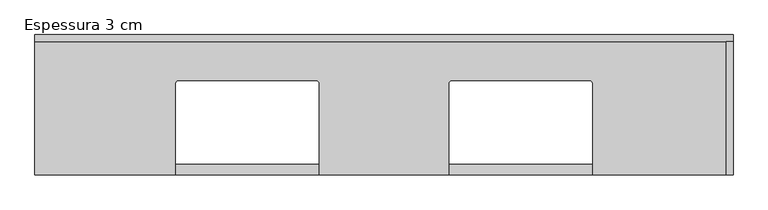
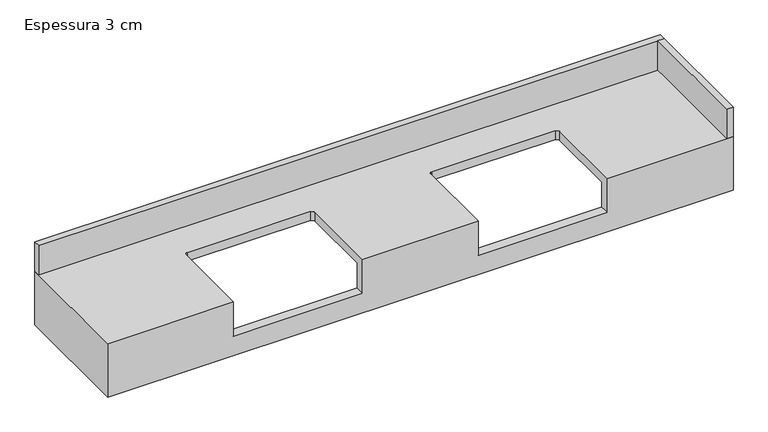
"""IFC4 building model written with IfcOpenShell, lengths in millimetres: furniture geometry, CC_BANCADA BANHEIRO COM DUAS CUBAS_CANTO RETO : Espessura 3 cm."""

from ifc_helpers import new_model, si_unit, frame, origin, place, context, project, spatial, polyline, circle_curve, outline, extrude, source, transform, mapped, element, save
from ifc_brep_helpers import plane_surface, revolved_surface, advanced_brep


def espessura_3_cm_cd586bec(model_context):
    return source(origin(), model_context, "Body", "SolidModel", [
        advanced_brep(
        [(750.0, 300.0, 860.0), (-1237.8, 300.0, 860.0), (-1237.8, -100.0, 860.0), (-837.8, -100.0, 860.0), (-837.8, 160.0, 860.0), (-827.8, 170.0, 860.0), (-437.8, 170.0, 860.0), (-427.8, 160.0, 860.0), (-427.8, -100.0, 860.0), (-60.0, -100.0, 860.0), (-60.0, 160.0, 860.0), (-50.0, 170.0, 860.0), (340.0, 170.0, 860.0), (350.0, 160.0, 860.0), (350.0, -100.0, 860.0), (750.0, -100.0, 860.0), (750.0, 300.0, 680.0), (720.0, 300.0, 680.0), (720.0, 300.0, 830.0), (-1207.8, 300.0, 830.0), (-1207.8, 300.0, 680.0), (-1237.8, 300.0, 680.0), (-1237.8, -100.0, 680.0), (750.0, -100.0, 680.0), (350.0, -100.0, 745.0), (-60.0, -100.0, 745.0), (-427.8, -100.0, 745.0), (-837.8, -100.0, 745.0), (720.0, -70.0, 830.0), (350.0, -70.0, 830.0), (350.0, 160.0, 830.0), (340.0, 170.0, 830.0), (-50.0, 170.0, 830.0), (-60.0, 160.0, 830.0), (-60.0, -70.0, 830.0), (-427.8, -70.0, 830.0), (-427.8, 160.0, 830.0), (-437.8, 170.0, 830.0), (-827.8, 170.0, 830.0), (-837.8, 160.0, 830.0), (-837.8, -70.0, 830.0), (-1207.8, -70.0, 830.0), (-1207.8, -70.0, 680.0), (-837.8, -70.0, 745.0), (-427.8, -70.0, 745.0), (-60.0, -70.0, 745.0), (350.0, -70.0, 745.0), (720.0, -70.0, 680.0)],
        [
            (0, 1),
            (1, 2),
            (2, 3),
            (3, 4),
            (4, 5, circle_curve(frame((-827.8, 160.0, 860.0), z_axis=(0.0, 0.0, -1.0), x_axis=(0.0, 1.0, 0.0)), 10.0)),
            (5, 6),
            (6, 7, circle_curve(frame((-437.8, 160.0, 860.0), z_axis=(0.0, 0.0, -1.0), x_axis=(0.0, 1.0, 0.0)), 10.0)),
            (7, 8),
            (8, 9),
            (9, 10),
            (10, 11, circle_curve(frame((-50.0, 160.0, 860.0), z_axis=(0.0, 0.0, -1.0), x_axis=(0.0, 1.0, 0.0)), 10.0)),
            (11, 12),
            (12, 13, circle_curve(frame((340.0, 160.0, 860.0), z_axis=(0.0, 0.0, -1.0), x_axis=(0.0, 1.0, 0.0)), 10.0)),
            (13, 14),
            (14, 15),
            (15, 0),
            (0, 16),
            (16, 17),
            (17, 18),
            (18, 19),
            (19, 20),
            (20, 21),
            (21, 1),
            (21, 22),
            (22, 2),
            (22, 23),
            (23, 15),
            (14, 24),
            (24, 25),
            (25, 9),
            (8, 26),
            (26, 27),
            (27, 3),
            (23, 16),
            (18, 28),
            (28, 29),
            (29, 30),
            (30, 31, circle_curve(frame((340.0, 160.0, 830.0), z_axis=(0.0, 0.0, 1.0), x_axis=(0.0, 1.0, 0.0)), 10.0)),
            (31, 32),
            (32, 33, circle_curve(frame((-50.0, 160.0, 830.0), z_axis=(0.0, 0.0, 1.0), x_axis=(0.0, 1.0, 0.0)), 10.0)),
            (33, 34),
            (34, 35),
            (35, 36),
            (36, 37, circle_curve(frame((-437.8, 160.0, 830.0), z_axis=(0.0, 0.0, 1.0), x_axis=(0.0, 1.0, 0.0)), 10.0)),
            (37, 38),
            (38, 39, circle_curve(frame((-827.8, 160.0, 830.0), z_axis=(0.0, 0.0, 1.0), x_axis=(0.0, 1.0, 0.0)), 10.0)),
            (39, 40),
            (40, 41),
            (41, 19),
            (41, 42),
            (42, 20),
            (40, 43),
            (43, 44),
            (44, 35),
            (34, 45),
            (45, 46),
            (46, 29),
            (28, 47),
            (47, 42),
            (17, 47),
            (5, 38),
            (37, 6),
            (26, 44),
            (43, 27),
            (4, 39),
            (7, 36),
            (24, 46),
            (45, 25),
            (11, 32),
            (31, 12),
            (10, 33),
            (13, 30),
        ],
        [
            plane_surface(frame((-1237.8, 300.0, 860.0), z_axis=(0.0, 0.0, 1.0), x_axis=(-1.0, 0.0, 0.0))),
            plane_surface(frame((750.0, 300.0, 860.0), z_axis=(0.0, 1.0, 0.0), x_axis=(0.0, 0.0, -1.0))),
            plane_surface(frame((-1237.8, 300.0, 860.0), z_axis=(-1.0, 0.0, 0.0), x_axis=(0.0, 0.0, -1.0))),
            plane_surface(frame((-1237.8, -100.0, 860.0), z_axis=(0.0, -1.0, 0.0), x_axis=(0.0, 0.0, -1.0))),
            plane_surface(frame((750.0, -100.0, 860.0), z_axis=(1.0, 0.0, 0.0), x_axis=(0.0, 0.0, -1.0))),
            plane_surface(frame((-1207.8, 300.0, 830.0), z_axis=(0.0, 0.0, -1.0), x_axis=(-1.0, 0.0, 0.0))),
            plane_surface(frame((-1207.8, 300.0, 830.0), z_axis=(1.0, 0.0, 0.0), x_axis=(0.0, 0.0, -1.0))),
            plane_surface(frame((-1207.8, -70.0, 830.0), z_axis=(0.0, 1.0, 0.0), x_axis=(0.0, 0.0, -1.0))),
            plane_surface(frame((720.0, -70.0, 830.0), z_axis=(-1.0, 0.0, 0.0), x_axis=(0.0, 0.0, -1.0))),
            plane_surface(frame((750.0, -100.0, 680.0), z_axis=(0.0, 0.0, -1.0), x_axis=(0.0, 1.0, 0.0))),
            plane_surface(frame((-827.8, 170.0, 745.0), z_axis=(0.0, -1.0, 0.0), x_axis=(0.0, 0.0, 1.0))),
            plane_surface(frame((-437.8, 170.0, 745.0), z_axis=(0.0, 0.0, 1.0), x_axis=(1.0, 0.0, 0.0))),
            revolved_surface(polyline([(-827.8, 170.0, 830.0), (-827.8, 170.0, 860.0)]), (-827.8, 160.0, 900.0), (0.0, 0.0, -1.0)),
            plane_surface(frame((-837.8, -230.0, 745.0), z_axis=(1.0, 0.0, 0.0), x_axis=(0.0, 0.0, 1.0))),
            plane_surface(frame((-427.8, 160.0, 745.0), z_axis=(-1.0, 0.0, 0.0), x_axis=(0.0, 0.0, 1.0))),
            revolved_surface(polyline([(-437.8, 170.0, 830.0), (-437.8, 170.0, 860.0)]), (-437.8, 160.0, 900.0), (0.0, 0.0, -1.0)),
            plane_surface(frame((340.0, 170.0, 745.0), z_axis=(0.0, 0.0, 1.0), x_axis=(1.0, 0.0, 0.0))),
            plane_surface(frame((-50.0, 170.0, 745.0), z_axis=(0.0, -1.0, 0.0), x_axis=(0.0, 0.0, 1.0))),
            revolved_surface(polyline([(-50.0, 170.0, 830.0), (-50.0, 170.0, 860.0)]), (-50.0, 160.0, 900.0), (0.0, 0.0, -1.0)),
            plane_surface(frame((-60.0, -230.0, 745.0), z_axis=(1.0, 0.0, 0.0), x_axis=(0.0, 0.0, 1.0))),
            plane_surface(frame((350.0, 160.0, 745.0), z_axis=(-1.0, 0.0, 0.0), x_axis=(0.0, 0.0, 1.0))),
            revolved_surface(polyline([(340.0, 170.0, 830.0), (340.0, 170.0, 860.0)]), (340.0, 160.0, 900.0), (0.0, 0.0, -1.0)),
        ],
        [
            (0, [[1, 2, 3, 4, 5, 6, 7, 8, 9, 10, 11, 12, 13, 14, 15, 16]]),
            (1, [[-1, 17, 18, 19, 20, 21, 22, 23]]),
            (2, [[-2, -23, 24, 25]]),
            (3, [[-3, -25, 26, 27, -15, 28, 29, 30, -9, 31, 32, 33]]),
            (4, [[-16, -27, 34, -17]]),
            (5, [[35, 36, 37, 38, 39, 40, 41, 42, 43, 44, 45, 46, 47, 48, 49, -20]]),
            (6, [[-49, 50, 51, -21]]),
            (7, [[-48, 52, 53, 54, -42, 55, 56, 57, -36, 58, 59, -50]]),
            (8, [[-35, -19, 60, -58]]),
            (9, [[-18, -34, -26, -24, -22, -51, -59, -60]]),
            (10, [[-6, 61, -45, 62]]),
            (11, [[-32, 63, -53, 64]]),
            (12, [[-5, 65, -46, -61]]),
            (13, [[-4, -33, -64, -52, -47, -65]]),
            (14, [[-8, 66, -43, -54, -63, -31]]),
            (15, [[-7, -62, -44, -66]]),
            (16, [[-29, 67, -56, 68]]),
            (17, [[-12, 69, -39, 70]]),
            (18, [[-11, 71, -40, -69]]),
            (19, [[-10, -30, -68, -55, -41, -71]]),
            (20, [[-14, 72, -37, -57, -67, -28]]),
            (21, [[-13, -70, -38, -72]]),
        ],
    ),
        extrude(outline(polyline([(730.0, 280.0), (750.0, 280.0), (750.0, -100.0), (730.0, -100.0), (730.0, 280.0)])), frame((0.0, 0.0, 860.0), z_axis=(0.0, 0.0, 1.0), x_axis=(1.0, 0.0, 0.0)), (0.0, 0.0, 1.0), 100.0),
        extrude(outline(polyline([(750.0, 300.0), (750.0, 280.0), (-1237.8, 280.0), (-1237.8, 300.0), (750.0, 300.0)])), frame((0.0, 0.0, 860.0), z_axis=(0.0, 0.0, 1.0), x_axis=(1.0, 0.0, 0.0)), (0.0, 0.0, 1.0), 100.0),
    ])


if __name__ == "__main__":
    model = new_model("IFC4")
    model_context = context("Model", 3, world=origin())
    ifc_project = project(units=[si_unit("LENGTHUNIT", "METRE", prefix="MILLI")], contexts=[model_context])
    site = spatial("IfcSite", under=ifc_project)
    building = spatial("IfcBuilding", under=site)
    placement = place(None, origin())
    espessura_3_cm_shape = espessura_3_cm_cd586bec(model_context)
    element("IfcFurniture", 1, ObjectType="CC_BANCADA BANHEIRO COM DUAS CUBAS_CANTO RETO : Espessura 3 cm", at=placement, inside=building, context=model_context, shape_type="MappedRepresentation", body=[
        mapped(espessura_3_cm_shape, transform((0.0, 0.0, 0.0), x_axis=(1.0, 0.0, 0.0), y_axis=(0.0, 1.0, 0.0), z_axis=(0.0, 0.0, 1.0))),
    ])
    save(model, "model.ifc")

# Revit data of these elements
# Type "CC_BANCADA BANHEIRO COM DUAS CUBAS_CANTO RETO : Espessura 3 cm"
#   Uso HS [instance default] = ""
#   h TESTEIRA AUX [instance default] = 0.15 m
#   Altura testeira [instance default] = 0.15 m
#   Altura rodapia [instance default] = 0.10 m
#   Espessura rodapia [instance default] = 0.02 m
#   Prof/2 [instance default] = 0.20 m
#   Offset cuba direita [instance default] = 0.40 m
#   Offset cuba esquerda [instance default] = 0.40 m
#   Depth [instance default] = 2.00 m
#   Width [instance default] = 0.40 m
#   Espessura bancada = 0.03 m
#   Comprimento [instance default] = 2.00 m
#   Height [instance default] = 0.86 m
#   Testeira [instance default] = yes
#   Rodapia fundo [instance default] = no
#   Rodapia esquerda [instance default] = no
#   Rodapia direita [instance default] = no
#   Material porta-toalha [instance default] = .CROMADO
#   Material hidráulico [instance default] = .CROMADO
#   Material cuba [instance default] = .PORCELANA BRANCA
#   Material bancada [instance default] = .GRANITO_BRANCO_ITAUNAS
#   Assembly Code = ""
# Element 1 (IfcFurniture, "CC_BANCADA BANHEIRO COM DUAS CUBAS_CANTO RETO : Espessura 3 cm")
#   Uso HS = "SUÍTE MASTER"
#   Depth = 1.9878 m
#   Comprimento = 1.9878 m
#   Rodapia fundo = yes
#   Rodapia direita = yes
#   Materials on its faces: ".GRANITO_BRANCO_ITAUNAS"
# Materials
#   ".CROMADO": class "CC_METAIS", colour RGB 211 223 226, transparency 0, Cost = 0
#   ".PORCELANA BRANCA": class "CC_PORCELANA", colour RGB 230 230 230, transparency 0, Cost = 0
#   ".GRANITO_BRANCO_ITAUNAS": class ".CC_PEDRA REVEST.", colour RGB 202 195 174, transparency 0, Description = "Revestimento em granito", Cost = 0
